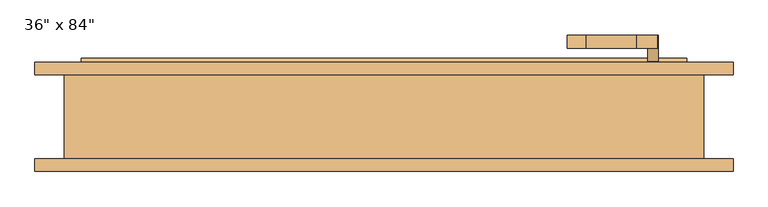
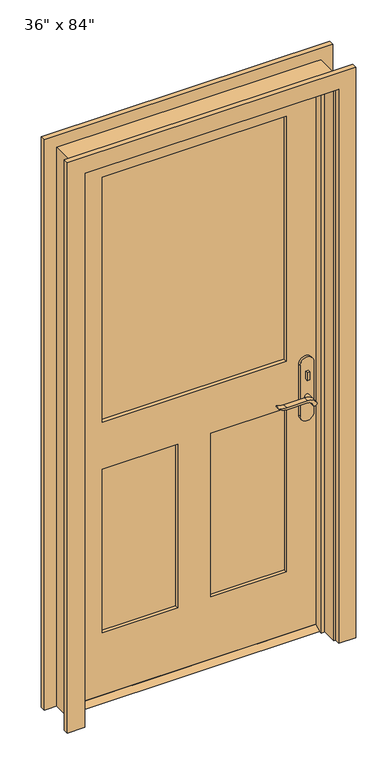
"""IFC4 building model written with IfcOpenShell, lengths in millimetres: door geometry."""

from ifc_helpers import new_model, si_unit, point, frame, frame_2d, origin, place, context, project, spatial, polyline, circle_curve, trimmed, segment, composite_curve, outline, extrude, faceted_brep, source, transform, mapped, element, save


def door_eeb9ac29(model_context):
    return source(origin(), model_context, "Body", "SolidModel", [
        extrude(outline(polyline([(25.4, 12.7), (60.325, 12.7), (85.725, 0.0), (0.0, 0.0), (25.4, 12.7)])), frame((-457.2, 0.0, 0.0), z_axis=(1.0, 0.0, 0.0), x_axis=(0.0, 1.0, 0.0)), (0.0, 0.0, 1.0), 914.4),
        extrude(outline(polyline([(411.4, 5.4), (401.4, 5.4), (401.4, 15.4), (411.4, 15.4), (411.4, 5.4)])), frame((0.0, 0.0, 981.9), z_axis=(0.0, 0.0, 1.0), x_axis=(1.0, 0.0, 0.0)), (0.0, 0.0, 1.0), 30.0),
        extrude(outline(composite_curve([segment(trimmed(circle_curve(frame_2d((996.9, 406.4)), 8.0), [point((996.9, 398.4))], [point((996.9, 414.4))], False, "CARTESIAN"), True, "CONTINUOUS"), segment(trimmed(circle_curve(frame_2d((996.9, 406.4)), 8.0), [point((996.9, 414.4))], [point((996.9, 398.4))], False, "CARTESIAN"), True, "CONTINUOUS")], self_intersect=False)), frame((0.0, 70.325, 0.0), z_axis=(0.0, 1.0, 0.0), x_axis=(0.0, 0.0, 1.0)), (0.0, 0.0, 1.0), 10.0),
        extrude(outline(composite_curve([segment(trimmed(circle_curve(frame_2d((897.1555521, 382.7324871)), 37.2832219), [point((919.0523287, 412.9081363))], [point((934.4, 381.0325667))], False, "CARTESIAN"), True, "CONTINUOUS"), segment(polyline([(934.4, 381.0325667), (934.4, 304.7564091)]), True, "CONTINUOUS"), segment(trimmed(circle_curve(frame_2d((1017.6850638, 304.8227909)), 83.2850902), [point((934.4, 304.7564091))], [point((939.4, 276.4))], True, "CARTESIAN"), True, "CONTINUOUS"), segment(polyline([(939.4, 276.4), (936.6135558, 276.4)]), True, "CONTINUOUS"), segment(trimmed(circle_curve(frame_2d((986.6709207, 308.3396612)), 59.3791355), [point((936.6135558, 276.4))], [point((927.4, 304.7564091))], False, "CARTESIAN"), True, "CONTINUOUS"), segment(polyline([(927.4, 304.7564091), (927.4, 381.0138099)]), True, "CONTINUOUS"), segment(trimmed(circle_curve(frame_2d((909.2738613, 381.0138099)), 18.1261387), [point((927.4, 381.0138099))], [point((914.4, 398.4))], True, "CARTESIAN"), True, "CONTINUOUS"), segment(trimmed(circle_curve(frame_2d((914.4, 406.4)), 8.0), [point((914.4, 398.4))], [point((919.0523287, 412.9081363))], False, "CARTESIAN"), True, "CONTINUOUS")], self_intersect=False)), frame((0.0, -34.6, 0.0), z_axis=(0.0, 1.0, 0.0), x_axis=(0.0, 0.0, 1.0)), (0.0, 0.0, 1.0), 20.0),
        extrude(outline(composite_curve([segment(trimmed(circle_curve(frame_2d((914.4, 406.4)), 8.0), [point((914.3999903, 398.4))], [point((919.0523287, 412.9081363))], False, "CARTESIAN"), True, "CONTINUOUS"), segment(trimmed(circle_curve(frame_2d((897.1555521, 382.7324871)), 37.2832219), [point((919.0523287, 412.9081363))], [point((934.4, 381.0325667))], False, "CARTESIAN"), True, "CONTINUOUS"), segment(polyline([(934.4, 381.0325667), (934.4, 304.7564091)]), True, "CONTINUOUS"), segment(trimmed(circle_curve(frame_2d((1017.6850638, 304.8227909)), 83.2850902), [point((934.4, 304.7564091))], [point((939.4, 276.4))], True, "CARTESIAN"), True, "CONTINUOUS"), segment(polyline([(939.4, 276.4), (936.6135558, 276.4)]), True, "CONTINUOUS"), segment(trimmed(circle_curve(frame_2d((986.6709207, 308.3396612)), 59.3791355), [point((936.6135558, 276.4))], [point((927.4, 304.7564091))], False, "CARTESIAN"), True, "CONTINUOUS"), segment(polyline([(927.4, 304.7564091), (927.4, 381.0138122)]), True, "CONTINUOUS"), segment(trimmed(circle_curve(frame_2d((909.2738682, 381.0138122)), 18.1261318), [point((927.4, 381.0138122))], [point((914.3999903, 398.4))], True, "CARTESIAN"), True, "CONTINUOUS")], self_intersect=False)), frame((0.0, 100.325, 0.0), z_axis=(0.0, 1.0, 0.0), x_axis=(0.0, 0.0, 1.0)), (0.0, 0.0, 1.0), 20.0),
        extrude(outline(composite_curve([segment(trimmed(circle_curve(frame_2d((914.4, 406.4)), 8.0), [point((914.4, 398.4))], [point((914.4, 414.4))], False, "CARTESIAN"), True, "CONTINUOUS"), segment(trimmed(circle_curve(frame_2d((914.4, 406.4)), 8.0), [point((914.4, 414.4))], [point((914.4, 398.4))], False, "CARTESIAN"), True, "CONTINUOUS")], self_intersect=False)), frame((0.0, -14.6, 0.0), z_axis=(0.0, 1.0, 0.0), x_axis=(0.0, 0.0, 1.0)), (0.0, 0.0, 1.0), 30.0),
        extrude(outline(composite_curve([segment(trimmed(circle_curve(frame_2d((914.4, 406.4)), 8.0), [point((914.4, 398.4))], [point((914.4, 414.4))], False, "CARTESIAN"), True, "CONTINUOUS"), segment(trimmed(circle_curve(frame_2d((914.4, 406.4)), 8.0), [point((914.4, 414.4))], [point((914.4, 398.4))], False, "CARTESIAN"), True, "CONTINUOUS")], self_intersect=False)), frame((0.0, 70.325, 0.0), z_axis=(0.0, 1.0, 0.0), x_axis=(0.0, 0.0, 1.0)), (0.0, 0.0, 1.0), 30.0),
        extrude(outline(composite_curve([segment(polyline([(844.4, 431.4), (1039.4, 431.4)]), True, "CONTINUOUS"), segment(trimmed(circle_curve(frame_2d((1039.4, 406.4)), 25.0), [point((1039.4, 431.4))], [point((1039.4, 381.4))], False, "CARTESIAN"), True, "CONTINUOUS"), segment(polyline([(1039.4, 381.4), (844.4, 381.4)]), True, "CONTINUOUS"), segment(trimmed(circle_curve(frame_2d((844.4, 406.4)), 25.0), [point((844.4, 381.4))], [point((844.4, 431.4))], False, "CARTESIAN"), True, "CONTINUOUS")], self_intersect=False)), frame((0.0, 15.4, 0.0), z_axis=(0.0, 1.0, 0.0), x_axis=(0.0, 0.0, 1.0)), (0.0, 0.0, 1.0), 10.0),
        extrude(outline(composite_curve([segment(polyline([(844.4, 431.4), (1039.4, 431.4)]), True, "CONTINUOUS"), segment(trimmed(circle_curve(frame_2d((1039.4, 406.4)), 25.0), [point((1039.4, 431.4))], [point((1039.4, 381.4))], False, "CARTESIAN"), True, "CONTINUOUS"), segment(polyline([(1039.4, 381.4), (844.4, 381.4)]), True, "CONTINUOUS"), segment(trimmed(circle_curve(frame_2d((844.4, 406.4)), 25.0), [point((844.4, 381.4))], [point((844.4, 431.4))], False, "CARTESIAN"), True, "CONTINUOUS")], self_intersect=False)), frame((0.0, 60.325, 0.0), z_axis=(0.0, 1.0, 0.0), x_axis=(0.0, 0.0, 1.0)), (0.0, 0.0, 1.0), 10.0),
        extrude(outline(polyline([(2133.6, -457.2), (12.7, -457.2), (12.7, 457.2), (2133.6, 457.2), (2133.6, -457.2)]), holes=[polyline([(1066.8, -336.55), (2012.95, -336.55), (2012.95, 336.55), (1066.8, 336.55), (1066.8, -336.55)]), polyline([(885.825, -60.325), (254.0, -60.325), (254.0, -336.55), (885.825, -336.55), (885.825, -60.325)]), polyline([(885.825, 336.55), (254.0, 336.55), (254.0, 60.325), (885.825, 60.325), (885.825, 336.55)])]), frame((0.0, 25.4, 0.0), z_axis=(0.0, 1.0, 0.0), x_axis=(0.0, 0.0, 1.0)), (0.0, 0.0, 1.0), 34.925),
        faceted_brep([(482.6, 60.325, 0.0), (482.6, -66.675, 0.0), (457.2, -66.675, 0.0), (457.2, -9.525, 0.0), (444.5, -9.525, 0.0), (444.5, 25.4, 0.0), (457.2, 25.4, 0.0), (457.2, 60.325, 0.0), (482.6, 60.325, 2159.0), (482.6, -66.675, 2159.0), (-482.6, -66.675, 2159.0), (-482.6, -66.675, 0.0), (-457.2, -66.675, 0.0), (-457.2, -66.675, 2133.6), (457.2, -66.675, 2133.6), (457.2, -9.525, 2133.6), (-457.2, -9.525, 2133.6), (-457.2, -9.525, 0.0), (-444.5, -9.525, 0.0), (-444.5, -9.525, 2120.9), (444.5, -9.525, 2120.9), (444.5, 25.4, 2120.9), (-444.5, 25.4, 2120.9), (-444.5, 25.4, 0.0), (-457.2, 25.4, 0.0), (-457.2, 25.4, 2133.6), (457.2, 25.4, 2133.6), (457.2, 60.325, 2133.6), (-457.2, 60.325, 2133.6), (-457.2, 60.325, 0.0), (-482.6, 60.325, 0.0), (-482.6, 60.325, 2159.0)], [[[0, 1, 2, 3, 4, 5, 6, 7]], [[1, 0, 8, 9]], [[2, 1, 9, 10, 11, 12, 13, 14]], [[3, 2, 14, 15]], [[4, 3, 15, 16, 17, 18, 19, 20]], [[5, 4, 20, 21]], [[6, 5, 21, 22, 23, 24, 25, 26]], [[7, 6, 26, 27]], [[0, 7, 27, 28, 29, 30, 31, 8]], [[9, 8, 31, 10]], [[15, 14, 13, 16]], [[21, 20, 19, 22]], [[27, 26, 25, 28]], [[30, 29, 24, 23, 18, 17, 12, 11]], [[10, 31, 30, 11]], [[16, 13, 12, 17]], [[22, 19, 18, 23]], [[28, 25, 24, 29]]]),
        extrude(outline(polyline([(-60.325, 37.0416667), (-336.55, 37.0416667), (-336.55, 48.6833333), (-60.325, 48.6833333), (-60.325, 37.0416667)])), frame((0.0, 0.0, 254.0), z_axis=(0.0, 0.0, 1.0), x_axis=(1.0, 0.0, 0.0)), (0.0, 0.0, 1.0), 631.825),
        extrude(outline(polyline([(336.55, 37.0416667), (60.325, 37.0416667), (60.325, 48.6833333), (336.55, 48.6833333), (336.55, 37.0416667)])), frame((0.0, 0.0, 254.0), z_axis=(0.0, 0.0, 1.0), x_axis=(1.0, 0.0, 0.0)), (0.0, 0.0, 1.0), 631.825),
        extrude(outline(polyline([(336.55, 39.37), (-336.55, 39.37), (-336.55, 46.355), (336.55, 46.355), (336.55, 39.37)])), frame((0.0, 0.0, 1066.8), z_axis=(0.0, 0.0, 1.0), x_axis=(1.0, 0.0, 0.0)), (0.0, 0.0, 1.0), 946.15),
        extrude(outline(polyline([(0.0, -527.05), (0.0, -463.55), (2139.95, -463.55), (2139.95, 463.55), (0.0, 463.55), (0.0, 527.05), (2203.45, 527.05), (2203.45, -527.05), (0.0, -527.05)])), frame((0.0, -85.725, 0.0), z_axis=(0.0, 1.0, 0.0), x_axis=(0.0, 0.0, 1.0)), (0.0, 0.0, 1.0), 19.05),
        extrude(outline(polyline([(0.0, -527.05), (0.0, -463.55), (2139.95, -463.55), (2139.95, 463.55), (0.0, 463.55), (0.0, 527.05), (2203.45, 527.05), (2203.45, -527.05), (0.0, -527.05)])), frame((0.0, 60.325, 0.0), z_axis=(0.0, 1.0, 0.0), x_axis=(0.0, 0.0, 1.0)), (0.0, 0.0, 1.0), 19.05),
    ])


if __name__ == "__main__":
    model = new_model("IFC4")
    model_context = context("Model", 3, world=origin())
    ifc_project = project(units=[si_unit("LENGTHUNIT", "METRE", prefix="MILLI")], contexts=[model_context])
    site = spatial("IfcSite", under=ifc_project)
    building = spatial("IfcBuilding", under=site)
    placement = place(None, origin())
    door_shape = door_eeb9ac29(model_context)
    element("IfcDoor", 1, ObjectType="Door-Exterior-Single-Entry-Half Flat Glass-Wood_Clad : 36\" x 84\"", at=placement, inside=building, context=model_context, shape_type="MappedRepresentation", body=[
        mapped(door_shape, transform((0.0, 0.0, 0.0), x_axis=(1.0, 0.0, 0.0), y_axis=(0.0, 1.0, 0.0), z_axis=(0.0, 0.0, 1.0))),
    ])
    save(model, "model.ifc")

# Revit data of these elements
# Type "Door-Exterior-Single-Entry-Half Flat Glass-Wood_Clad : 36\" x 84\""
#   Type Mark = "aa"
#   Assembly Code = "B2030100"
#   Analytic Construction = "French door, wood frame with single glass"
#   Top Rail = 0' - 4 3/4"
#   Threshold Offset [instance default] = 0' - 0 1/2"
#   Thickness = 0' - 1 3/8"
#   Thermal Resistance (R) = 0.188367 (m²·K)/W
#   Swing Angle [instance default] = 90.00°
#   Stiles = 0' - 4 3/4"
#   Rough Width = 3' - 2"
#   Rough Height = 7' - 1"
#   Lock Rail = 0' - 7 1/8"
#   Height = 7' - 0"
#   Width = 3' - 0"
#   Heat Transfer Coefficient (U) = 5.30918 W/(m²·K)
#   Door Offset [instance default] = 0' - 0"
#   Bottom Rail = 0' - 9 1/2"
#   Threshold [instance default] = yes
#   Function = 1
#   Exterior Trim [instance default] = yes
#   Trim Material = Trim
#   Threshold Material = Cherry
#   Panel Material = Trim
#   Glazing = EXISTING WINDOW
#   Frame Material = Trim
#   Door Handle Material = Aluminum
#   Visual Light Transmittance = 0
#   Solar Heat Gain Coefficient = 0
#   Wall Closure = (empty or 0)
#   Construction Type = (empty or 0)
# Element 1 (IfcDoor, "Door-Exterior-Single-Entry-Half Flat Glass-Wood_Clad : 36\" x 84\"")
#   Materials on its faces: "Trim", "Aluminum", "Cherry", "EXISTING WINDOW"
# Materials
#   "Trim": class "Wood", colour RGB 250 251 245, transparency 0, Cost = 0
#   "Cherry": class "Wood", colour RGB 154 107 61, transparency 0, Description = "Prunus Serotina", Cost = 0
#   "EXISTING WINDOW": class "Glass", colour RGB 218 227 224, transparency 0.85, Description = "Soda Lime Glass", Cost = 0
#   "Aluminum": class "Metal", colour RGB 244 244 244, transparency 0, Description = "Aluminum 6061", Cost = 0
